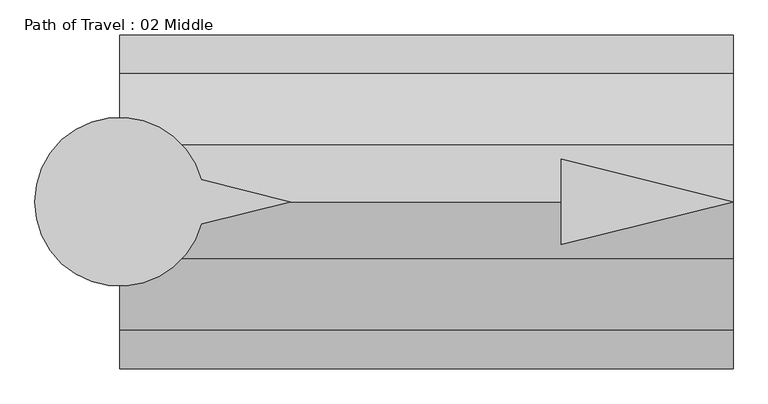
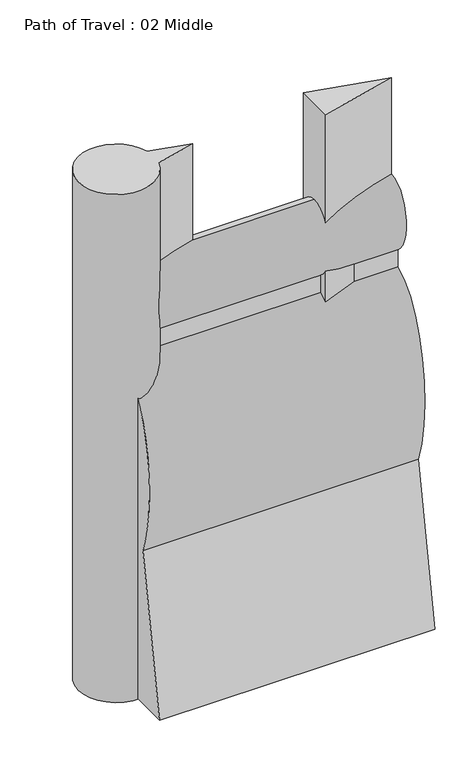
"""IFC4 building model written with IfcOpenShell, lengths in millimetres: proxy geometry, Path of Travel : 02 Middle."""

from ifc_helpers import new_model, si_unit, point, frame, frame_2d, origin, origin_with_axes, place, context, project, spatial, polyline, circle_curve, ellipse_curve, trimmed, segment, composite_curve, outline, extrude, source, transform, mapped, element, save
from ifc_brep_helpers import plane_surface, extruded_surface, advanced_brep


def path_of_travel_02_middle_3345a40d(model_context):
    return source(origin(), model_context, "Body", "SolidModel", [
        advanced_brep(
        [(227.5554837, 0.0, 1727.2), (227.5554837, 42.9018657, 1436.6534209), (227.5554837, 42.9018657, 1363.4763406), (227.5554837, 184.1186263, 643.4144547), (227.5554837, 297.5699544, 0.0), (227.5554837, 145.6574193, 0.0), (227.5554837, 0.0, 584.2), (227.5554837, -145.6574193, 0.0), (227.5554837, -297.5699544, 0.0), (227.5554837, -184.1186263, 643.4144547), (227.5554837, -42.9018657, 1363.4763406), (227.5554837, -42.9018657, 1436.6534209), (1319.7554837, 0.0, 1727.2), (1319.7554837, -42.9018657, 1436.6534209), (1319.7554837, -42.9018657, 1363.4763406), (1319.7554837, -184.1186263, 643.4144547), (1319.7554837, -297.5699544, 0.0), (1319.7554837, -145.6574193, 0.0), (1319.7554837, 0.0, 584.2), (1319.7554837, 145.6574193, 0.0), (1319.7554837, 297.5699544, 0.0), (1319.7554837, 184.1186263, 643.4144547), (1319.7554837, 42.9018657, 1363.4763406), (1319.7554837, 42.9018657, 1436.6534209)],
        [
            (0, 1, ellipse_curve(frame((227.5554837, 0.0, 1574.8), z_axis=(-1.0, 0.0, 0.0), x_axis=(0.0, 0.0, 1.0)), 152.4, 101.6)),
            (1, 2),
            (2, 3, ellipse_curve(frame((227.5554837, 0.0, 914.4), z_axis=(-1.0, 0.0, 0.0), x_axis=(0.0, 0.0, -1.0)), 457.2, 228.6)),
            (3, 4),
            (4, 5),
            (5, 6),
            (6, 7),
            (7, 8),
            (8, 9),
            (9, 10, ellipse_curve(frame((227.5554837, 0.0, 914.4), z_axis=(-1.0, 0.0, 0.0), x_axis=(0.0, 0.0, -1.0)), 457.2, 228.6)),
            (10, 11),
            (11, 0, ellipse_curve(frame((227.5554837, 0.0, 1574.8), z_axis=(-1.0, 0.0, 0.0), x_axis=(0.0, 0.0, 1.0)), 152.4, 101.6)),
            (12, 13, ellipse_curve(frame((1319.7554837, 0.0, 1574.8), z_axis=(1.0, 0.0, 0.0), x_axis=(0.0, 0.0, 1.0)), 152.4, 101.6)),
            (13, 14),
            (14, 15, ellipse_curve(frame((1319.7554837, 0.0, 914.4), z_axis=(1.0, 0.0, 0.0), x_axis=(0.0, 0.0, -1.0)), 457.2, 228.6)),
            (15, 16),
            (16, 17),
            (17, 18),
            (18, 19),
            (19, 20),
            (20, 21),
            (21, 22, ellipse_curve(frame((1319.7554837, 0.0, 914.4), z_axis=(1.0, 0.0, 0.0), x_axis=(0.0, 0.0, -1.0)), 457.2, 228.6)),
            (22, 23),
            (23, 12, ellipse_curve(frame((1319.7554837, 0.0, 1574.8), z_axis=(1.0, 0.0, 0.0), x_axis=(0.0, 0.0, 1.0)), 152.4, 101.6)),
            (0, 12),
            (23, 1),
            (22, 2),
            (21, 3),
            (20, 4),
            (19, 5),
            (18, 6),
            (17, 7),
            (16, 8),
            (15, 9),
            (14, 10),
            (13, 11),
        ],
        [
            plane_surface(frame((227.5554837, 0.0, 0.0), z_axis=(-1.0, 0.0, 0.0), x_axis=(0.0, 0.0, 1.0))),
            plane_surface(frame((1319.7554837, 0.0, 0.0), z_axis=(1.0, 0.0, 0.0), x_axis=(0.0, 0.0, 1.0))),
            extruded_surface(trimmed(ellipse_curve(frame((1319.7554837, 0.0, 1574.8), z_axis=(-1.0, 0.0, 0.0), x_axis=(0.0, 0.0, 1.0)), 152.4, 101.6), [point((1319.7554837, 0.0, 1727.2))], [point((1319.7554837, 42.9018657, 1436.6534209))], True, "CARTESIAN"), (-1092.2, 0.0, 0.0), 1092.2),
            plane_surface(frame((227.5554837, 42.9018657, 1436.6534209), z_axis=(0.0, 1.0, 0.0), x_axis=(1.0, 0.0, 0.0))),
            extruded_surface(trimmed(ellipse_curve(frame((1319.7554837, 0.0, 914.4), z_axis=(-1.0, 0.0, 0.0), x_axis=(0.0, 0.0, -1.0)), 457.2, 228.6), [point((1319.7554837, 42.9018657, 1363.4763406))], [point((1319.7554837, 184.1186263, 643.4144547))], True, "CARTESIAN"), (-1092.2, 0.0, 0.0), 1092.2),
            plane_surface(frame((227.5554837, 184.1186263, 643.4144547), z_axis=(0.0, 0.9848077530122078, 0.1736481776669322), x_axis=(1.0, 0.0, 0.0))),
            plane_surface(frame((227.5554837, 297.5699544, 0.0), z_axis=(0.0, 0.0, -1.0), x_axis=(1.0, 0.0, 0.0))),
            plane_surface(frame((227.5554837, 145.6574193, 0.0), z_axis=(0.0, -0.9702957262760199, -0.2419218955995739), x_axis=(1.0, 0.0, 0.0))),
            plane_surface(frame((227.5554837, 0.0, 584.2), z_axis=(0.0, 0.9702957262759961, -0.24192189559966923), x_axis=(1.0, 0.0, 0.0))),
            plane_surface(frame((227.5554837, -145.6574193, 0.0), z_axis=(0.0, 0.0, -1.0), x_axis=(1.0, 0.0, 0.0))),
            plane_surface(frame((227.5554837, -297.5699544, 0.0), z_axis=(0.0, -0.984807753012208, 0.17364817766693066), x_axis=(1.0, 0.0, 0.0))),
            extruded_surface(trimmed(ellipse_curve(frame((1319.7554837, 0.0, 914.4), z_axis=(-1.0, 0.0, 0.0), x_axis=(0.0, 0.0, -1.0)), 457.2, 228.6), [point((1319.7554837, -184.1186263, 643.4144547))], [point((1319.7554837, -42.9018657, 1363.4763406))], True, "CARTESIAN"), (-1092.2, 0.0, 0.0), 1092.2),
            plane_surface(frame((227.5554837, -42.9018657, 1363.4763406), z_axis=(0.0, -1.0, 0.0), x_axis=(1.0, 0.0, 0.0))),
            extruded_surface(trimmed(ellipse_curve(frame((1319.7554837, 0.0, 1574.8), z_axis=(-1.0, 0.0, 0.0), x_axis=(0.0, 0.0, 1.0)), 152.4, 101.6), [point((1319.7554837, -42.9018657, 1436.6534209))], [point((1319.7554837, 0.0, 1727.2))], True, "CARTESIAN"), (-1092.2, 0.0, 0.0), 1092.2),
        ],
        [
            (0, [[1, 2, 3, 4, 5, 6, 7, 8, 9, 10, 11, 12]]),
            (1, [[13, 14, 15, 16, 17, 18, 19, 20, 21, 22, 23, 24]]),
            (2, [[-1, 25, -24, 26]]),
            (3, [[-2, -26, -23, 27]]),
            (4, [[-3, -27, -22, 28]]),
            (5, [[-4, -28, -21, 29]]),
            (6, [[-5, -29, -20, 30]]),
            (7, [[-6, -30, -19, 31]]),
            (8, [[-7, -31, -18, 32]]),
            (9, [[-8, -32, -17, 33]]),
            (10, [[-9, -33, -16, 34]]),
            (11, [[-10, -34, -15, 35]]),
            (12, [[-11, -35, -14, 36]]),
            (13, [[-12, -36, -13, -25]]),
        ],
    ),
        extrude(outline(polyline([(1013.7503371, 76.2006338), (1319.7554837, 0.0), (1013.7503371, -76.2006338), (1013.7503371, 76.2006338)])), origin_with_axes(), (0.0, 0.0, 1.0), 2129.5973753),
        extrude(outline(composite_curve([segment(polyline([(372.7837828, 39.4440225), (531.182385, 0.0), (372.7837828, -39.4440225)]), True, "CONTINUOUS"), segment(trimmed(circle_curve(frame_2d((227.2200886, 0.0)), 150.8131956), [point((372.7837828, -39.4440225))], [point((372.7837828, 39.4440225))], False, "CARTESIAN"), True, "CONTINUOUS")], self_intersect=False)), origin_with_axes(), (0.0, 0.0, 1.0), 2129.5973753),
    ])


if __name__ == "__main__":
    model = new_model("IFC4")
    model_context = context("Model", 3, world=origin())
    ifc_project = project(units=[si_unit("LENGTHUNIT", "METRE", prefix="MILLI")], contexts=[model_context])
    site = spatial("IfcSite", under=ifc_project)
    building = spatial("IfcBuilding", under=site)
    placement = place(None, origin())
    path_of_travel_02_middle_shape = path_of_travel_02_middle_3345a40d(model_context)
    element("IfcBuildingElementProxy", 1, Name="Path of Travel : 02 Middle", ObjectType="Path of Travel : 02 Middle", at=placement, inside=building, context=model_context, shape_type="MappedRepresentation", body=[
        mapped(path_of_travel_02_middle_shape, transform((0.0, 0.0, 0.0), x_axis=(1.0, 0.0, 0.0), y_axis=(0.0, 1.0, 0.0), z_axis=(0.0, 0.0, 1.0))),
    ])
    save(model, "model.ifc")

# Revit data of these elements
# Type "Path of Travel : 02 Middle"
#   Path of Egress [instance default] = 4' - 0"
#   built-in parameter 1001306 [instance default] = 4 (stored number, unit not read)
#   Dot at Start = no
#   Arrow in Middle = yes
#   Arrow at End = no
#   Egress Path = none
# Element 1 (IfcBuildingElementProxy, "Path of Travel : 02 Middle")
#   Path of Egress = 3' - 7"
#   built-in parameter 1001306 = 3.58333 (stored number, unit not read)
#   Materials on its faces: "Egress Path Solid", "solid"
# Materials
#   "Egress Path Solid": class "Unassigned", colour RGB 255 128 64, transparency 0.75, Comments = "Rendering appearance not upgraded "
#   "solid": class "Generic", colour RGB 120 120 120, transparency 0, Cost = 0
